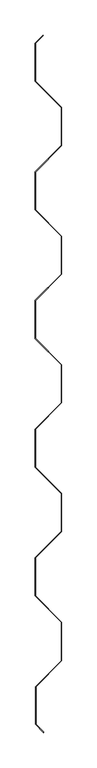
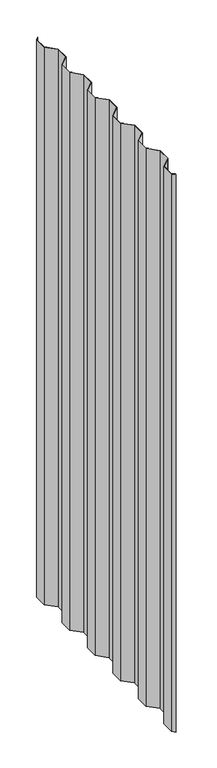
"""IFC4 building model written with IfcOpenShell, lengths in millimetres: proxy geometry, MBCI 7.2-V Panel17 : MBCI 7.2-V Panel-1."""

from ifc_helpers import new_model, si_unit, origin, origin_with_axes, place, context, project, spatial, polyline, outline, extrude, source, transform, mapped, element, save


def generic_models_c7c5b5ce(model_context):
    return source(origin(), model_context, "Body", "SweptSolid", [
        extrude(outline(polyline([(590353.5827614, -534354.3919067), (590353.5827614, -534300.2801976), (590364.9833956, -534288.8795634), (590365.0253204, -534289.6795376), (590354.1780739, -534300.5267841), (590354.1780739, -534354.1453202), (590391.6684739, -534391.6357202), (590391.6684739, -534445.9163841), (590354.1780739, -534483.4067841), (590354.1780739, -534537.0253202), (590391.6684739, -534574.5157202), (590391.6684739, -534628.7963841), (590354.1780739, -534666.2867841), (590354.1780739, -534719.9053202), (590391.6684739, -534757.3957202), (590391.6684739, -534811.6763841), (590354.1780739, -534849.1667841), (590354.1780739, -534902.7853202), (590391.6684739, -534940.2757202), (590391.6684739, -534994.5563841), (590354.1780739, -535032.0467841), (590354.1780739, -535085.6653202), (590391.6684739, -535123.1557202), (590391.6684739, -535178.2999841), (590354.7876739, -535215.1807841), (590354.7876739, -535268.2689111), (590365.9181078, -535279.399345), (590365.8630841, -535280.1862203), (590354.1923614, -535268.5154976), (590354.1923614, -535214.9341976), (590391.0731614, -535178.0533976), (590391.0731614, -535123.4023067), (590353.5827614, -535085.9119067), (590353.5827614, -535031.8001976), (590391.0731614, -534994.3097976), (590391.0731614, -534940.5223067), (590353.5827614, -534903.0319067), (590353.5827614, -534848.9201976), (590391.0731614, -534811.4297976), (590391.0731614, -534757.6423067), (590353.5827614, -534720.1519067), (590353.5827614, -534666.0401976), (590391.0731614, -534628.5497976), (590391.0731614, -534574.7623067), (590353.5827614, -534537.2719067), (590353.5827614, -534483.1601976), (590391.0731614, -534445.6697976), (590391.0731614, -534391.8823067), (590353.5827614, -534354.3919067)])), origin_with_axes(), (0.0, 0.0, 1.0), 2438.4),
    ])


if __name__ == "__main__":
    model = new_model("IFC4")
    model_context = context("Model", 3, world=origin())
    ifc_project = project(units=[si_unit("LENGTHUNIT", "METRE", prefix="MILLI")], contexts=[model_context])
    site = spatial("IfcSite", under=ifc_project)
    building = spatial("IfcBuilding", under=site)
    placement = place(None, origin())
    generic_models_shape = generic_models_c7c5b5ce(model_context)
    element("IfcBuildingElementProxy", 1, Name="MBCI 7.2-V Panel17 : MBCI 7.2-V Panel-1", ObjectType="MBCI 7.2-V Panel17 : MBCI 7.2-V Panel-1", at=placement, inside=building, context=model_context, shape_type="MappedRepresentation", body=[
        mapped(generic_models_shape, transform((0.0, 0.0, 0.0), x_axis=(1.0, 0.0, 0.0), y_axis=(0.0, 1.0, 0.0), z_axis=(0.0, 0.0, 1.0))),
    ])
    save(model, "model.ifc")

# Revit data of these elements
# Element 1 (IfcBuildingElementProxy, "MBCI 7.2-V Panel17 : MBCI 7.2-V Panel-1")
#   Materials on its faces: "MTL PANEL"
# Materials
#   "MTL PANEL": class "Generic", colour RGB 239 242 240, transparency 0, Cost = 0
